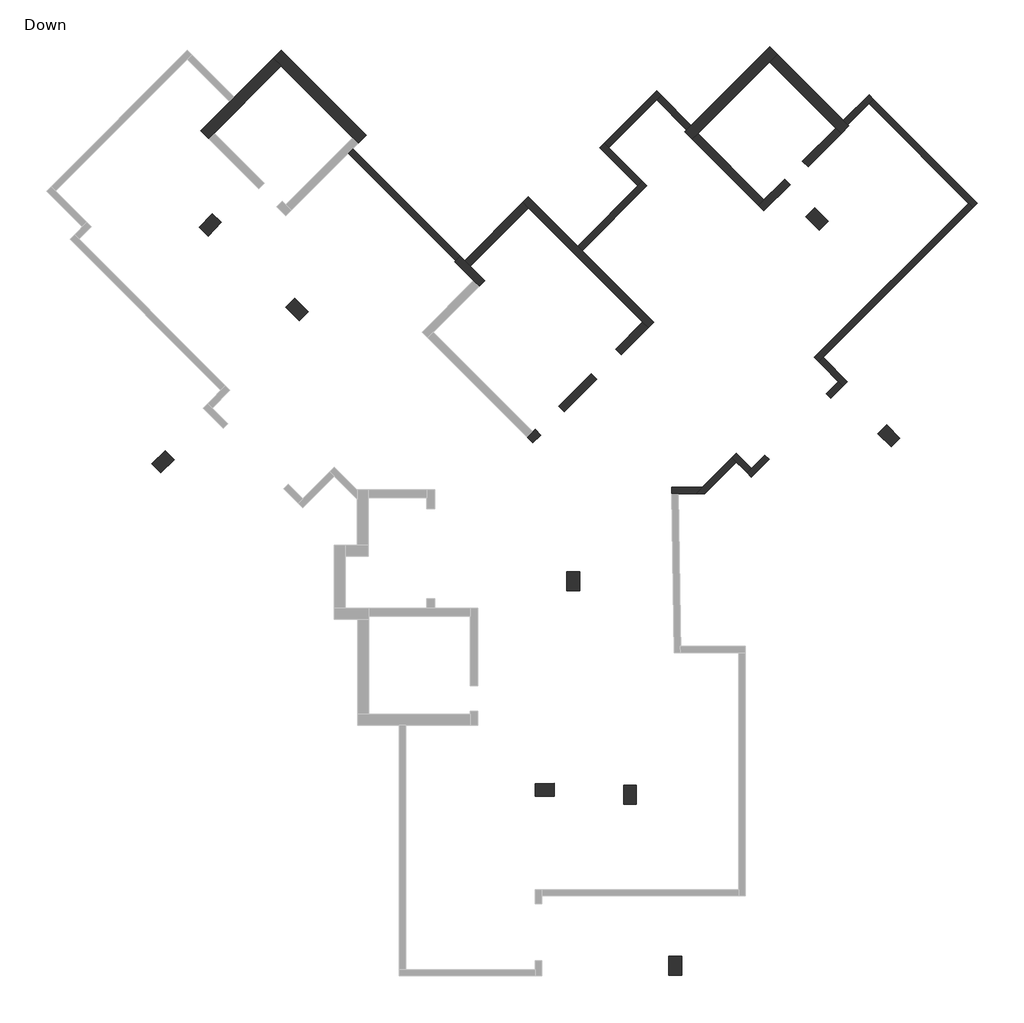
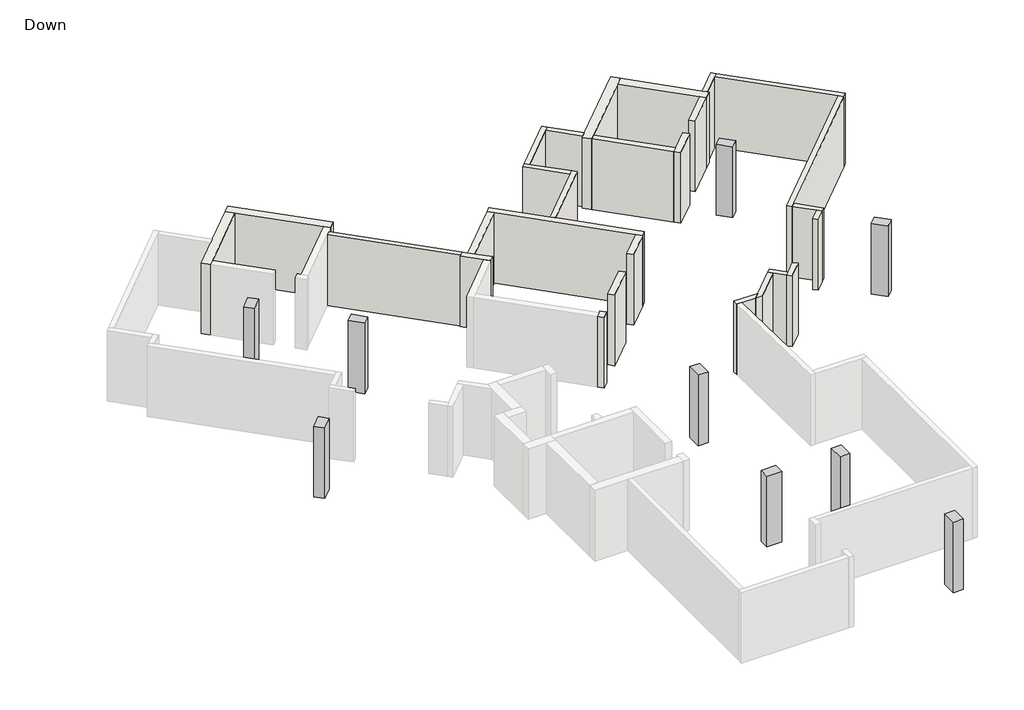
# One storey, part 2 of 2: 27 walls, 9 columns.
"""IFC4 building model written with IfcOpenShell, lengths in millimetres."""

from ifc_helpers import new_model, si_unit, origin, origin_with_axes, place, context, project, spatial, polyline, outline, extrude, faceted_brep, element, save

model = new_model("IFC4")

# Units and contexts
model_context = context("Model", 3, world=origin())
ifc_project = project(units=[si_unit("LENGTHUNIT", "METRE", prefix="MILLI")], contexts=[model_context])

# Site, building, storey
site = spatial("IfcSite", under=ifc_project)
building = spatial("IfcBuilding", under=site)
storey = spatial("IfcBuildingStorey", under=building, Name="Down", Elevation=0.0)

# Columns
placement = place(None, origin())
element("IfcColumn", 1, ObjectType="Concrete Rectengular Column : 40/60", at=placement, inside=storey, context=model_context, shape_type="SweptSolid", body=[
    extrude(outline(polyline([(6112.9804297, -13069.1556852), (6112.9804297, -13669.1556852), (5712.9804297, -13669.1556852), (5712.9804297, -13069.1556852), (6112.9804297, -13069.1556852)])), origin_with_axes(), (0.0, 0.0, 1.0), 3000.0),
])
element("IfcColumn", 2, ObjectType="Concrete Rectengular Column : 40/60", at=placement, inside=storey, context=model_context, shape_type="Brep", body=[
    faceted_brep([(4677.0922421, -7661.9946197, 0.0), (4677.0922421, -8261.9946197, 0.0), (4277.0922421, -8261.9946197, 0.0), (4277.0922421, -7661.9946197, 0.0), (4677.0922421, -7661.9946197, 3000.0), (4677.0922421, -8261.9946197, 3000.0), (4677.0922421, -8261.9946197, 2820.0), (4677.0922421, -7661.9946197, 2820.0), (4277.0922421, -8261.9946197, 3000.0), (4277.0922421, -8261.9946197, 2820.0), (4277.0922421, -7661.9946197, 3000.0), (4277.0922421, -7661.9946197, 2820.0)], [[[0, 1, 2, 3]], [[4, 5, 6, 1, 0, 7]], [[5, 8, 9, 2, 1, 6]], [[8, 10, 11, 3, 2, 9]], [[10, 4, 7, 0, 3, 11]], [[4, 10, 8, 5]]]),
])
element("IfcColumn", 3, ObjectType="Concrete Rectengular Column : 40/60", at=placement, inside=storey, context=model_context, shape_type="Brep", body=[
    faceted_brep([(2484.8469761, -1497.4694814, 0.0), (2484.8469761, -897.4694814, 0.0), (2884.8469761, -897.4694814, 0.0), (2884.8469761, -1497.4694814, 0.0), (2484.8469761, -1497.4694814, 3000.0), (2484.8469761, -897.4694814, 3000.0), (2484.8469761, -897.4694814, 2820.0), (2484.8469761, -1497.4694814, 2820.0), (2884.8469761, -897.4694814, 3000.0), (2884.8469761, -897.4694814, 2820.0), (2884.8469761, -1497.4694814, 3000.0), (2884.8469761, -1497.4694814, 2820.0)], [[[0, 1, 2, 3]], [[4, 5, 6, 1, 0, 7]], [[5, 8, 9, 2, 1, 6]], [[8, 10, 11, 3, 2, 9]], [[10, 4, 7, 0, 3, 11]], [[4, 10, 8, 5]]]),
])
element("IfcColumn", 4, ObjectType="Concrete Rectengular Column : 40/60", at=placement, inside=storey, context=model_context, shape_type="Brep", body=[
    faceted_brep([(-6125.9760682, 7745.4646162, 0.0), (-5702.252807, 7320.6604284, 0.0), (-5985.4555989, 7038.1782543, 0.0), (-6409.17886, 7462.9824421, 0.0), (-6125.9760682, 7745.4646162, 3000.0), (-5702.252807, 7320.6604284, 3000.0), (-5702.252807, 7320.6604284, 2820.0), (-6125.9760682, 7745.4646162, 2820.0), (-5985.4555989, 7038.1782543, 3000.0), (-5985.4555989, 7038.1782543, 2820.0), (-6409.17886, 7462.9824421, 3000.0), (-6409.17886, 7462.9824421, 2820.0)], [[[0, 1, 2, 3]], [[4, 5, 6, 1, 0, 7]], [[5, 8, 9, 2, 1, 6]], [[8, 10, 11, 3, 2, 9]], [[10, 4, 7, 0, 3, 11]], [[4, 10, 8, 5]]]),
])
element("IfcColumn", 5, ObjectType="Concrete Rectengular Column : 40/60", at=placement, inside=storey, context=model_context, shape_type="Brep", body=[
    faceted_brep([(1484.675203, -7607.3508739, 0.0), (2084.6127194, -7598.6919819, 0.0), (2090.385314, -7998.6503262, 0.0), (1490.4477976, -8007.3092182, 0.0), (1484.675203, -7607.3508739, 3000.0), (2084.6127194, -7598.6919819, 3000.0), (2084.6127194, -7598.6919819, 2820.0), (1484.675203, -7607.3508739, 2820.0), (2090.385314, -7998.6503262, 3000.0), (2090.385314, -7998.6503262, 2820.0), (1490.4477976, -8007.3092182, 3000.0), (1490.4477976, -8007.3092182, 2820.0)], [[[0, 1, 2, 3]], [[4, 5, 6, 1, 0, 7]], [[5, 8, 9, 2, 1, 6]], [[8, 10, 11, 3, 2, 9]], [[10, 4, 7, 0, 3, 11]], [[4, 10, 8, 5]]]),
])
element("IfcColumn", 6, ObjectType="Concrete Rectengular Column : 40/60", at=placement, inside=storey, context=model_context, shape_type="Brep", body=[
    faceted_brep([(10319.9156396, 10604.3419273, 0.0), (10744.1797083, 10180.0778586, 0.0), (10461.3369958, 9897.2351461, 0.0), (10037.0729271, 10321.4992148, 0.0), (10319.9156396, 10604.3419273, 3000.0), (10744.1797083, 10180.0778586, 3000.0), (10744.1797083, 10180.0778586, 2820.0), (10319.9156396, 10604.3419273, 2820.0), (10461.3369958, 9897.2351461, 3000.0), (10461.3369958, 9897.2351461, 2820.0), (10037.0729271, 10321.4992148, 3000.0), (10037.0729271, 10321.4992148, 2820.0)], [[[0, 1, 2, 3]], [[4, 5, 6, 1, 0, 7]], [[5, 8, 9, 2, 1, 6]], [[8, 10, 11, 3, 2, 9]], [[10, 4, 7, 0, 3, 11]], [[4, 10, 8, 5]]]),
])
element("IfcColumn", 7, ObjectType="Concrete Rectengular Column : 40/60", at=placement, inside=storey, context=model_context, shape_type="Brep", body=[
    faceted_brep([(-8440.7447422, 10142.7112538, 0.0), (-8856.8048079, 9710.3988417, 0.0), (-9145.0130827, 9987.7722189, 0.0), (-8728.9530169, 10420.084631, 0.0), (-8440.7447422, 10142.7112538, 3000.0), (-8856.8048079, 9710.3988417, 3000.0), (-8856.8048079, 9710.3988417, 2820.0), (-8440.7447422, 10142.7112538, 2820.0), (-9145.0130827, 9987.7722189, 3000.0), (-9145.0130827, 9987.7722189, 2820.0), (-8728.9530169, 10420.084631, 3000.0), (-8728.9530169, 10420.084631, 2820.0)], [[[0, 1, 2, 3]], [[4, 5, 6, 1, 0, 7]], [[5, 8, 9, 2, 1, 6]], [[8, 10, 11, 3, 2, 9]], [[10, 4, 7, 0, 3, 11]], [[4, 10, 8, 5]]]),
])
element("IfcColumn", 8, ObjectType="Concrete Rectengular Column : 40/60", at=placement, inside=storey, context=model_context, shape_type="Brep", body=[
    faceted_brep([(-9937.9307713, 2645.0605261, 0.0), (-10362.7349591, 2221.337265, 0.0), (-10645.2171332, 2504.5400569, 0.0), (-10220.4129454, 2928.263318, 0.0), (-9937.9307713, 2645.0605261, 3000.0), (-10362.7349591, 2221.337265, 3000.0), (-10362.7349591, 2221.337265, 2820.0), (-9937.9307713, 2645.0605261, 2820.0), (-10643.7250884, 2503.0442058, 3000.0), (-10645.2171332, 2504.5400569, 3000.0), (-10220.4129454, 2928.263318, 3000.0), (-10219.2939768, 2927.1414948, 3000.0)], [[[0, 1, 2, 3]], [[4, 5, 6, 1, 0, 7]], [[5, 8, 9, 2, 1, 6]], [[9, 10, 3, 2]], [[10, 11, 4, 7, 0, 3]], [[4, 11, 10, 9, 8, 5]]]),
])
element("IfcColumn", 9, ObjectType="Concrete Rectengular Column : 40/60", at=placement, inside=storey, context=model_context, shape_type="SweptSolid", body=[
    extrude(outline(polyline([(12593.7668598, 3749.362272), (13018.0309285, 3325.0982033), (12735.188216, 3042.2554908), (12310.9241473, 3466.5195596), (12593.7668598, 3749.362272)])), origin_with_axes(), (0.0, 0.0, 1.0), 3000.0),
])

# Walls
element("IfcWall", 10, ObjectType="20", at=placement, inside=storey, context=model_context, shape_type="Brep", body=[
    faceted_brep([(-4429.582499, 12332.1948217, 0.0), (-1033.4026062, 8936.0149288, 0.0), (-1033.4026062, 8936.0149288, 2820.0), (-1033.4026062, 8936.0149288, 3000.0), (-4429.582499, 12332.1948217, 3000.0), (-4429.582499, 12332.1948217, 2820.0), (-4288.1611428, 12473.6161779, 0.0), (-4288.1611428, 12473.6161779, 3000.0), (-891.98125, 9077.4362851, 3000.0), (-891.98125, 9077.4362851, 0.0)], [[[0, 1, 2, 3, 4, 5]], [[6, 7, 8, 9]], [[1, 0, 6, 9]], [[3, 2, 1, 9, 8]], [[4, 3, 8, 7]], [[0, 5, 4, 7, 6]]]),
])
element("IfcWall", 11, ObjectType="20", at=placement, inside=storey, context=model_context, shape_type="Brep", body=[
    faceted_brep([(2962.7877192, 9255.2480262, 0.0), (5013.5473558, 11306.0076628, 0.0), (5013.5473558, 11306.0076628, 2820.0), (5013.5473558, 11306.0076628, 3000.0), (2962.7877192, 9255.2480262, 3000.0), (2962.7877192, 9255.2480262, 2820.0), (2821.3663629, 9396.6693825, 0.0), (2821.3663629, 9396.6693825, 3000.0), (4730.7046433, 11306.0076628, 3000.0), (4872.1259995, 11447.429019, 3000.0), (4872.1259995, 11447.429019, 0.0), (4730.7046433, 11306.0076628, 0.0)], [[[0, 1, 2, 3, 4, 5]], [[6, 7, 8, 9, 10, 11]], [[1, 0, 6, 11, 10]], [[4, 3, 9, 8, 7]], [[0, 5, 4, 7, 6]], [[3, 2, 1, 10, 9]]]),
])
element("IfcWall", 12, ObjectType="20", at=placement, inside=storey, context=model_context, shape_type="Brep", body=[
    faceted_brep([(4872.1259995, 11447.429019, 0.0), (3807.7763909, 12511.7786276, 0.0), (3666.3550347, 12653.1999839, 0.0), (3666.3550347, 12653.1999839, 3000.0), (3807.7763909, 12511.7786276, 3000.0), (4872.1259995, 11447.429019, 3000.0), (4730.7046433, 11306.0076628, 0.0), (4730.7046433, 11306.0076628, 3000.0), (3524.9336785, 12511.7786276, 3000.0), (3524.9336785, 12511.7786276, 0.0)], [[[0, 1, 2, 3, 4, 5]], [[6, 7, 8, 9]], [[2, 1, 0, 6, 9]], [[5, 4, 3, 8, 7]], [[0, 5, 7, 6]], [[3, 2, 9, 8]]]),
])
element("IfcWall", 13, ObjectType="20", at=placement, inside=storey, context=model_context, shape_type="Brep", body=[
    faceted_brep([(3807.7763909, 12511.7786276, 0.0), (5320.554821, 14024.5570577, 0.0), (5461.9761772, 14165.978414, 0.0), (5461.9761772, 14165.978414, 3000.0), (5320.554821, 14024.5570577, 3000.0), (3807.7763909, 12511.7786276, 3000.0), (3807.7763909, 12511.7786276, 2820.0), (3666.3550347, 12653.1999839, 0.0), (3666.3550347, 12653.1999839, 3000.0), (5320.554821, 14307.3997702, 3000.0), (5320.554821, 14307.3997702, 0.0)], [[[0, 1, 2, 3, 4, 5, 6]], [[7, 8, 9, 10]], [[2, 1, 0, 7, 10]], [[5, 4, 3, 9, 8]], [[3, 2, 10, 9]], [[0, 6, 5, 8, 7]]]),
])
element("IfcWall", 14, ObjectType="20", at=placement, inside=storey, context=model_context, shape_type="Brep", body=[
    faceted_brep([(5320.554821, 14024.5570577, 0.0), (6266.9603358, 13078.1515429, 0.0), (6266.9603358, 13078.1515429, 2820.0), (6266.9603358, 13078.1515429, 3000.0), (5320.554821, 14024.5570577, 3000.0), (5320.554821, 14024.5570577, 2820.0), (5461.9761772, 14165.978414, 0.0), (5461.9761772, 14165.978414, 3000.0), (6408.3816921, 13219.5728991, 3000.0), (6408.3816921, 13219.5728991, 0.0)], [[[0, 1, 2, 3, 4, 5]], [[6, 7, 8, 9]], [[1, 0, 6, 9]], [[4, 3, 8, 7]], [[0, 5, 4, 7, 6]], [[3, 2, 1, 9, 8]]]),
])
element("IfcWall", 15, ObjectType="20", at=placement, inside=storey, context=model_context, shape_type="Brep", body=[
    faceted_brep([(11369.6407399, 13231.4427963, 0.0), (12039.7613133, 13901.5633697, 0.0), (12181.1826696, 14042.9847259, 0.0), (12181.1826696, 14042.9847259, 3000.0), (12039.7613133, 13901.5633697, 3000.0), (11369.6407399, 13231.4427963, 3000.0), (11369.6407399, 13231.4427963, 2820.0), (11228.2193837, 13372.8641525, 0.0), (11228.2193837, 13372.8641525, 3000.0), (12039.7613133, 14184.4060822, 3000.0), (12039.7613133, 14184.4060822, 0.0)], [[[0, 1, 2, 3, 4, 5, 6]], [[7, 8, 9, 10]], [[2, 1, 0, 7, 10]], [[5, 4, 3, 9, 8]], [[0, 6, 5, 8, 7]], [[3, 2, 10, 9]]]),
])
element("IfcWall", 16, ObjectType="20", at=placement, inside=storey, context=model_context, shape_type="Brep", body=[
    faceted_brep([(12039.7613133, 13901.5633697, 0.0), (15186.314453, 10755.0102301, 0.0), (15327.7358092, 10613.5888738, 0.0), (15327.7358092, 10613.5888738, 3000.0), (15186.314453, 10755.0102301, 3000.0), (12039.7613133, 13901.5633697, 3000.0), (12039.7613133, 13901.5633697, 2820.0), (12181.1826696, 14042.9847259, 0.0), (12181.1826696, 14042.9847259, 3000.0), (15469.1571655, 10755.0102301, 3000.0), (15469.1571655, 10755.0102301, 0.0)], [[[0, 1, 2, 3, 4, 5, 6]], [[7, 8, 9, 10]], [[2, 1, 0, 7, 10]], [[5, 4, 3, 9, 8]], [[0, 6, 5, 8, 7]], [[3, 2, 10, 9]]]),
])
element("IfcWall", 17, ObjectType="20", at=placement, inside=storey, context=model_context, shape_type="Brep", body=[
    faceted_brep([(15186.314453, 10755.0102301, 0.0), (10305.5209453, 5874.2167224, 0.0), (10305.5209453, 5874.2167224, 2820.0), (10305.5209453, 5874.2167224, 3000.0), (15186.314453, 10755.0102301, 3000.0), (15186.314453, 10755.0102301, 2820.0), (10446.9423016, 5732.7953662, 0.0), (10588.3636578, 5874.2167224, 0.0), (15327.7358092, 10613.5888738, 0.0), (15327.7358092, 10613.5888738, 3000.0), (10588.3636578, 5874.2167224, 3000.0), (10446.9423016, 5732.7953662, 3000.0)], [[[0, 1, 2, 3, 4, 5]], [[6, 7, 8, 9, 10, 11]], [[1, 0, 8, 7, 6]], [[4, 3, 11, 10, 9]], [[0, 5, 4, 9, 8]], [[3, 2, 1, 6, 11]]]),
])
element("IfcWall", 18, ObjectType="20", at=placement, inside=storey, context=model_context, shape_type="Brep", body=[
    faceted_brep([(10446.9423016, 5732.7953662, 0.0), (11069.4524151, 5110.2852526, 0.0), (11210.8737714, 4968.8638964, 0.0), (11210.8737714, 4968.8638964, 3000.0), (11069.4524151, 5110.2852526, 3000.0), (10446.9423016, 5732.7953662, 3000.0), (10588.3636578, 5874.2167224, 0.0), (10588.3636578, 5874.2167224, 3000.0), (11352.2951276, 5110.2852526, 3000.0), (11352.2951276, 5110.2852526, 0.0), (11292.5695034, 5050.5596284, 3000.0)], [[[0, 1, 2, 3, 4, 5]], [[6, 7, 8, 9]], [[2, 1, 0, 6, 9]], [[5, 4, 3, 10, 8, 7]], [[0, 5, 7, 6]], [[3, 2, 9, 8, 10]]]),
])
element("IfcWall", 19, ObjectType="20", at=placement, inside=storey, context=model_context, shape_type="Brep", body=[
    faceted_brep([(11069.4524151, 5110.2852526, 0.0), (10685.5360235, 4726.368861, 0.0), (10685.5360235, 4726.368861, 2820.0), (10685.5360235, 4726.368861, 3000.0), (11069.4524151, 5110.2852526, 3000.0), (11069.4524151, 5110.2852526, 2820.0), (11210.8737714, 4968.8638964, 0.0), (11210.8737714, 4968.8638964, 3000.0), (10826.9573797, 4584.9475048, 3000.0), (10826.9573797, 4584.9475048, 2820.0), (10826.9573797, 4584.9475048, 0.0)], [[[0, 1, 2, 3, 4, 5]], [[6, 7, 8, 9, 10]], [[1, 0, 6, 10]], [[3, 2, 1, 10, 9, 8]], [[4, 3, 8, 7]], [[0, 5, 4, 7, 6]]]),
])
element("IfcWall", 20, ObjectType="20", at=placement, inside=storey, context=model_context, shape_type="Brep", body=[
    faceted_brep([(8747.3931582, 2788.2259957, 0.0), (8323.1290895, 2363.961927, 0.0), (8181.7077332, 2222.5405707, 0.0), (8181.7077332, 2222.5405707, 3000.0), (8323.1290895, 2363.961927, 3000.0), (8747.3931582, 2788.2259957, 3000.0), (8747.3931582, 2788.2259957, 2820.0), (8888.8145144, 2646.8046394, 0.0), (8888.8145144, 2646.8046394, 2820.0), (8888.8145144, 2646.8046394, 3000.0), (8393.4317005, 2151.4218256, 3000.0), (8323.1290895, 2081.1192145, 3000.0), (8323.1290895, 2081.1192145, 0.0)], [[[0, 1, 2, 3, 4, 5, 6]], [[7, 8, 9, 10, 11, 12]], [[2, 1, 0, 7, 12]], [[5, 4, 3, 11, 10, 9]], [[0, 6, 5, 9, 8, 7]], [[3, 2, 12, 11]]]),
])
element("IfcWall", 21, ObjectType="20", at=placement, inside=storey, context=model_context, shape_type="Brep", body=[
    faceted_brep([(8323.1290895, 2363.961927, 0.0), (7842.9320868, 2844.1589296, 0.0), (7842.9320868, 2844.1589296, 2820.0), (7842.9320868, 2844.1589296, 3000.0), (8323.1290895, 2363.961927, 3000.0), (8323.1290895, 2363.961927, 2820.0), (8181.7077332, 2222.5405707, 0.0), (8181.7077332, 2222.5405707, 3000.0), (7842.9320868, 2561.3162171, 3000.0), (7701.5107306, 2702.7375734, 3000.0), (7701.5107306, 2702.7375734, 0.0), (7842.9320868, 2561.3162171, 0.0)], [[[0, 1, 2, 3, 4, 5]], [[6, 7, 8, 9, 10, 11]], [[1, 0, 6, 11, 10]], [[4, 3, 9, 8, 7]], [[0, 5, 4, 7, 6]], [[3, 2, 1, 10, 9]]]),
])
element("IfcWall", 22, ObjectType="20", at=placement, inside=storey, context=model_context, shape_type="Brep", body=[
    faceted_brep([(7701.5107306, 2702.7375734, 0.0), (6767.6697714, 1768.8966142, 0.0), (6567.6697714, 1568.8966142, 0.0), (6567.6697714, 1568.8966142, 3000.0), (6767.6697714, 1768.8966142, 3000.0), (7701.5107306, 2702.7375734, 3000.0), (7842.9320868, 2561.3162171, 0.0), (7842.9320868, 2561.3162171, 3000.0), (6850.5124839, 1568.8966142, 3000.0), (6850.5124839, 1568.8966142, 0.0)], [[[0, 1, 2, 3, 4, 5]], [[6, 7, 8, 9]], [[2, 1, 0, 6, 9]], [[5, 4, 3, 8, 7]], [[0, 5, 7, 6]], [[3, 2, 9, 8]]]),
])
element("IfcWall", 23, ObjectType="20", at=placement, inside=storey, context=model_context, shape_type="Brep", body=[
    faceted_brep([(6767.6697714, 1768.8966142, 0.0), (5805.6765523, 1768.8966142, 0.0), (5805.6765523, 1768.8966142, 2820.0), (5805.6765523, 1768.8966142, 3000.0), (6767.6697714, 1768.8966142, 3000.0), (6767.6697714, 1768.8966142, 2820.0), (6567.6697714, 1568.8966142, 0.0), (6567.6697714, 1568.8966142, 3000.0), (6008.5087812, 1568.8966142, 3000.0), (5808.4890075, 1568.8966142, 3000.0), (5808.4890075, 1568.8966142, 0.0), (6008.5087812, 1568.8966142, 0.0)], [[[0, 1, 2, 3, 4, 5]], [[6, 7, 8, 9, 10, 11]], [[1, 0, 6, 11, 10]], [[4, 3, 9, 8, 7]], [[0, 5, 4, 7, 6]], [[3, 2, 1, 10, 9]]]),
])
element("IfcWall", 24, ObjectType="25", at=placement, inside=storey, context=model_context, shape_type="Brep", body=[
    faceted_brep([(10980.691113, 13125.4176764, 0.0), (9934.0396226, 12078.766186, 0.0), (9934.0396226, 12078.766186, 2820.0), (9934.0396226, 12078.766186, 3000.0), (10980.691113, 13125.4176764, 3000.0), (10980.691113, 13125.4176764, 2820.0), (11157.4678083, 12948.6409811, 0.0), (11157.4678083, 12948.6409811, 3000.0), (10110.8163179, 11901.9894907, 3000.0), (10110.8163179, 11901.9894907, 2820.0), (10110.8163179, 11901.9894907, 0.0)], [[[0, 1, 2, 3, 4, 5]], [[6, 7, 8, 9, 10]], [[1, 0, 6, 10]], [[3, 2, 1, 10, 9, 8]], [[4, 3, 8, 7]], [[0, 5, 4, 7, 6]]]),
])
element("IfcWall", 25, ObjectType="25", at=placement, inside=storey, context=model_context, shape_type="Brep", body=[
    faceted_brep([(8717.8496812, 10509.0228541, 0.0), (9546.3438201, 11337.5169929, 0.0), (9546.3438201, 11337.5169929, 2820.0), (9546.3438201, 11337.5169929, 3000.0), (8717.8496812, 10509.0228541, 3000.0), (8717.8496812, 10509.0228541, 2820.0), (8541.0729859, 10685.7995493, 0.0), (8541.0729859, 10685.7995493, 3000.0), (8717.8496812, 10862.5762446, 3000.0), (9369.5671248, 11514.2936882, 3000.0), (9369.5671248, 11514.2936882, 2820.0), (9369.5671248, 11514.2936882, 0.0), (8717.8496812, 10862.5762446, 0.0)], [[[0, 1, 2, 3, 4, 5]], [[6, 7, 8, 9, 10, 11, 12]], [[1, 0, 6, 12, 11]], [[3, 2, 1, 11, 10, 9]], [[4, 3, 9, 8, 7]], [[0, 5, 4, 7, 6]]]),
])
element("IfcWall", 26, ObjectType="25", at=placement, inside=storey, context=model_context, shape_type="Brep", body=[
    faceted_brep([(8717.8496812, 10862.5762446, 0.0), (6632.1047328, 12948.3211931, 0.0), (6632.1047328, 12948.3211931, 2820.0), (6632.1047328, 12948.3211931, 3000.0), (8717.8496812, 10862.5762446, 3000.0), (8717.8496812, 10862.5762446, 2820.0), (8541.0729859, 10685.7995493, 0.0), (8541.0729859, 10685.7995493, 3000.0), (6455.3280375, 12771.5444978, 3000.0), (6455.3280375, 12771.5444978, 0.0)], [[[0, 1, 2, 3, 4, 5]], [[6, 7, 8, 9]], [[1, 0, 6, 9]], [[4, 3, 8, 7]], [[3, 2, 1, 9, 8]], [[0, 5, 4, 7, 6]]]),
])
element("IfcWall", 27, ObjectType="25", at=placement, inside=storey, context=model_context, shape_type="Brep", body=[
    faceted_brep([(5227.1373278, 6990.8984176, 0.0), (2962.7877192, 9255.2480262, 0.0), (2821.3663629, 9396.6693825, 0.0), (1265.7304614, 10952.305284, 0.0), (1265.7304614, 10952.305284, 3000.0), (2821.3663629, 9396.6693825, 3000.0), (2962.7877192, 9255.2480262, 3000.0), (5227.1373278, 6990.8984176, 3000.0), (5227.1373278, 6990.8984176, 2820.0), (5050.3606325, 6814.1217223, 0.0), (5050.3606325, 6814.1217223, 3000.0), (4873.5839372, 6990.8984176, 3000.0), (1265.7304614, 10598.7518934, 3000.0), (1088.9537661, 10775.5285887, 3000.0), (1088.9537661, 10775.5285887, 0.0), (1265.7304614, 10598.7518934, 0.0), (4873.5839372, 6990.8984176, 0.0)], [[[0, 1, 2, 3, 4, 5, 6, 7, 8]], [[9, 10, 11, 12, 13, 14, 15, 16]], [[3, 2, 1, 0, 9, 16, 15, 14]], [[7, 6, 5, 4, 13, 12, 11, 10]], [[4, 3, 14, 13]], [[0, 8, 7, 10, 9]]]),
])
element("IfcWall", 28, ObjectType="25", at=placement, inside=storey, context=model_context, shape_type="SweptSolid", body=[
    extrude(outline(polyline([(-750.5003772, 8936.0744454), (1088.9537661, 10775.5285887), (1265.7304614, 10598.7518934), (-573.7236819, 8759.2977501), (-750.5003772, 8936.0744454)])), origin_with_axes(), (0.0, 0.0, 1.0), 3000.0),
])
element("IfcWall", 29, ObjectType="25", at=placement, inside=storey, context=model_context, shape_type="Brep", body=[
    faceted_brep([(-115.3333666, 8300.9074348, 0.0), (-573.7236819, 8759.2977501, 0.0), (-750.5003772, 8936.0744454, 0.0), (-891.9217334, 9077.4958016, 0.0), (-891.9217334, 9077.4958016, 3000.0), (-750.5003772, 8936.0744454, 3000.0), (-573.7236819, 8759.2977501, 3000.0), (-115.3333666, 8300.9074348, 3000.0), (-292.1100618, 8124.1307395, 0.0), (-292.1100618, 8124.1307395, 3000.0), (-468.8867571, 8300.9074348, 3000.0), (-1068.6984287, 8900.7191063, 3000.0), (-1068.6984287, 8900.7191063, 2820.0), (-1068.6984287, 8900.7191063, 0.0), (-468.8867571, 8300.9074348, 0.0), (-1033.4026062, 8936.0149288, 0.0), (-1033.4026062, 8936.0149288, 3000.0)], [[[0, 1, 2, 3, 4, 5, 6, 7]], [[8, 9, 10, 11, 12, 13, 14]], [[3, 2, 1, 0, 8, 14, 13, 15]], [[4, 3, 15, 13, 12, 11, 16]], [[7, 6, 5, 4, 16, 11, 10, 9]], [[0, 7, 9, 8]]]),
])
element("IfcWall", 30, ObjectType="25", at=placement, inside=storey, context=model_context, shape_type="Brep", body=[
    faceted_brep([(1407.8225017, 3171.5835916, 0.0), (1655.2707813, 3419.0318712, 0.0), (1655.2707813, 3419.0318712, 2820.0), (1655.2707813, 3419.0318712, 3000.0), (1407.8225017, 3171.5835916, 3000.0), (1407.8225017, 3171.5835916, 2820.0), (1231.0458064, 3348.3602869, 0.0), (1231.0458064, 3348.3602869, 3000.0), (1407.8225017, 3525.1369821, 3000.0), (1478.494086, 3595.8085665, 3000.0), (1478.494086, 3595.8085665, 2820.0), (1478.494086, 3595.8085665, 0.0), (1407.8225017, 3525.1369821, 0.0)], [[[0, 1, 2, 3, 4, 5]], [[6, 7, 8, 9, 10, 11, 12]], [[1, 0, 6, 12, 11]], [[3, 2, 1, 11, 10, 9]], [[4, 3, 9, 8, 7]], [[0, 5, 4, 7, 6]]]),
])
element("IfcWall", 31, ObjectType="25", at=placement, inside=storey, context=model_context, shape_type="Brep", body=[
    faceted_brep([(2397.561133, 4161.3222229, 0.0), (3424.432188, 5188.1932779, 0.0), (3424.432188, 5188.1932779, 2820.0), (3424.432188, 5188.1932779, 3000.0), (2397.561133, 4161.3222229, 3000.0), (2397.561133, 4161.3222229, 2820.0), (2220.7844377, 4338.0989181, 0.0), (2220.7844377, 4338.0989181, 2820.0), (2220.7844377, 4338.0989181, 3000.0), (3247.6554927, 5364.9699732, 3000.0), (3247.6554927, 5364.9699732, 2820.0), (3247.6554927, 5364.9699732, 0.0)], [[[0, 1, 2, 3, 4, 5]], [[6, 7, 8, 9, 10, 11]], [[1, 0, 6, 11]], [[3, 2, 1, 11, 10, 9]], [[4, 3, 9, 8]], [[0, 5, 4, 8, 7, 6]]]),
])
element("IfcWall", 32, ObjectType="25", at=placement, inside=storey, context=model_context, shape_type="Brep", body=[
    faceted_brep([(4199.1842169, 5962.9453067, 0.0), (5050.3606325, 6814.1217223, 0.0), (5050.3606325, 6814.1217223, 3000.0), (4199.1842169, 5962.9453067, 3000.0), (4199.1842169, 5962.9453067, 2820.0), (4022.4075216, 6139.722002, 0.0), (4022.4075216, 6139.722002, 2820.0), (4022.4075216, 6139.722002, 3000.0), (4873.5839372, 6990.8984176, 3000.0), (4873.5839372, 6990.8984176, 0.0)], [[[0, 1, 2, 3, 4]], [[5, 6, 7, 8, 9]], [[1, 0, 5, 9]], [[3, 2, 8, 7]], [[0, 4, 3, 7, 6, 5]], [[2, 1, 9, 8]]]),
])
element("IfcWall", 33, ObjectType="35", at=placement, inside=storey, context=model_context, shape_type="Brep", body=[
    faceted_brep([(-6797.446529, 15338.5417926, 0.0), (-6549.9591555, 15091.0544192, 0.0), (-4287.1177238, 12828.2129875, 0.0), (-4110.3410285, 12651.4362922, 0.0), (-4110.3410285, 12651.4362922, 3000.0), (-4287.1177238, 12828.2129875, 3000.0), (-6549.9591555, 15091.0544192, 3000.0), (-6797.446529, 15338.5417926, 3000.0), (-6549.9591555, 15586.029166, 0.0), (-6549.9591555, 15586.029166, 3000.0), (-3862.8536551, 12898.9236656, 3000.0), (-3862.8536551, 12898.9236656, 0.0)], [[[0, 1, 2, 3, 4, 5, 6, 7]], [[8, 9, 10, 11]], [[3, 2, 1, 0, 8, 11]], [[7, 6, 5, 4, 10, 9]], [[0, 7, 9, 8]], [[4, 3, 11, 10]]]),
])
element("IfcWall", 34, ObjectType="35", at=placement, inside=storey, context=model_context, shape_type="Brep", body=[
    faceted_brep([(-6797.446529, 15338.5417926, 0.0), (-8031.9823439, 14104.0059776, 0.0), (-8173.4037002, 13962.5846214, 0.0), (-9095.6760176, 13040.312304, 0.0), (-9095.6760176, 13040.312304, 2820.0), (-9095.6760176, 13040.312304, 3000.0), (-8173.4037002, 13962.5846214, 3000.0), (-8031.9823439, 14104.0059776, 3000.0), (-6797.446529, 15338.5417926, 3000.0), (-6549.9591555, 15091.0544192, 0.0), (-6549.9591555, 15091.0544192, 2820.0), (-6549.9591555, 15091.0544192, 3000.0), (-8671.4119489, 12969.6016259, 3000.0), (-8848.1886442, 12792.8249306, 3000.0), (-8848.1886442, 12792.8249306, 0.0), (-8671.4119489, 12969.6016259, 0.0)], [[[0, 1, 2, 3, 4, 5, 6, 7, 8]], [[9, 10, 11, 12, 13, 14, 15]], [[3, 2, 1, 0, 9, 15, 14]], [[8, 7, 6, 5, 13, 12, 11]], [[0, 8, 11, 10, 9]], [[5, 4, 3, 14, 13]]]),
])
element("IfcWall", 35, ObjectType="35", at=placement, inside=storey, context=model_context, shape_type="Brep", body=[
    faceted_brep([(6455.3280375, 12771.5444978, 0.0), (6632.1047328, 12948.3211931, 0.0), (8894.9461646, 15211.1626248, 0.0), (9142.433538, 15458.6499982, 0.0), (9142.433538, 15458.6499982, 3000.0), (8894.9461646, 15211.1626248, 3000.0), (6632.1047328, 12948.3211931, 3000.0), (6455.3280375, 12771.5444978, 3000.0), (6207.8406641, 13019.0318712, 0.0), (6207.8406641, 13019.0318712, 2820.0), (6207.8406641, 13019.0318712, 3000.0), (6266.9603358, 13078.1515429, 3000.0), (6408.3816921, 13219.5728991, 3000.0), (8894.9461646, 15706.1373716, 3000.0), (8894.9461646, 15706.1373716, 0.0), (6408.3816921, 13219.5728991, 0.0), (6266.9603358, 13078.1515429, 0.0)], [[[0, 1, 2, 3, 4, 5, 6, 7]], [[8, 9, 10, 11, 12, 13, 14, 15, 16]], [[3, 2, 1, 0, 8, 16, 15, 14]], [[7, 6, 5, 4, 13, 12, 11, 10]], [[4, 3, 14, 13]], [[0, 7, 10, 9, 8]]]),
])
element("IfcWall", 36, ObjectType="35", at=placement, inside=storey, context=model_context, shape_type="Brep", body=[
    faceted_brep([(8894.9461646, 15211.1626248, 0.0), (10980.691113, 13125.4176764, 0.0), (11157.4678083, 12948.6409811, 0.0), (11157.4678083, 12948.6409811, 3000.0), (10980.691113, 13125.4176764, 3000.0), (8894.9461646, 15211.1626248, 3000.0), (8894.9461646, 15211.1626248, 2820.0), (9142.433538, 15458.6499982, 0.0), (9142.433538, 15458.6499982, 3000.0), (11228.2193837, 13372.8641525, 3000.0), (11369.6407399, 13231.4427963, 3000.0), (11404.9551817, 13196.1283545, 3000.0), (11404.9551817, 13196.1283545, 2820.0), (11404.9551817, 13196.1283545, 0.0), (11369.6407399, 13231.4427963, 0.0), (11228.2193837, 13372.8641525, 0.0)], [[[0, 1, 2, 3, 4, 5, 6]], [[7, 8, 9, 10, 11, 12, 13, 14, 15]], [[2, 1, 0, 7, 15, 14, 13]], [[5, 4, 3, 11, 10, 9, 8]], [[0, 6, 5, 8, 7]], [[3, 2, 13, 12, 11]]]),
])

save(model, "model.ifc")

# Revit data of these elements
# Type "Concrete Rectengular Column : 40/60"
#   b = 40 cm
#   h = 60 cm
#   Structural Material [instance default] = Concrete
# Type "20"
#   Layers, outside or top first: 20 cm "Concrete" (function 1)
# Type "25"
#   Layers, outside or top first: 25 cm "Concrete" (function 1)
# Type "35"
#   Layers, outside or top first: 35 cm "Concrete" (function 1)
# Element 1 (IfcColumn, "Concrete Rectengular Column : 40/60")
#   Comments = ""
#   Mark = "C1"
#   SOFiSTiK_AMG_Comments = ""
#   SOFiSTiK_AMG_Scheduled = yes
#   SOFiSTiK_AMG_Adjusted = yes
#   Structural Material = Concrete
#   Phase Created = New Construction
#   Materials on its faces: "Concrete"
# Element 2 (IfcColumn, "Concrete Rectengular Column : 40/60")
#   Comments = ""
#   Mark = "C2"
#   SOFiSTiK_AMG_Comments = ""
#   SOFiSTiK_AMG_Scheduled = yes
#   SOFiSTiK_AMG_Adjusted = yes
#   Structural Material = Concrete
#   Phase Created = New Construction
#   Materials on its faces: "Concrete"
# Element 3 (IfcColumn, "Concrete Rectengular Column : 40/60")
#   Comments = ""
#   Mark = "C3"
#   SOFiSTiK_AMG_Comments = ""
#   SOFiSTiK_AMG_Scheduled = yes
#   SOFiSTiK_AMG_Adjusted = yes
#   Structural Material = Concrete
#   Phase Created = New Construction
#   Materials on its faces: "Concrete"
# Element 4 (IfcColumn, "Concrete Rectengular Column : 40/60")
#   Comments = ""
#   Mark = "C4"
#   SOFiSTiK_AMG_Comments = ""
#   SOFiSTiK_AMG_Scheduled = yes
#   SOFiSTiK_AMG_Adjusted = yes
#   Structural Material = Concrete
#   Phase Created = New Construction
#   Materials on its faces: "Concrete"
# Element 5 (IfcColumn, "Concrete Rectengular Column : 40/60")
#   Comments = ""
#   Mark = "C5"
#   SOFiSTiK_AMG_Comments = ""
#   SOFiSTiK_AMG_Scheduled = yes
#   SOFiSTiK_AMG_Adjusted = yes
#   Structural Material = Concrete
#   Phase Created = New Construction
#   Materials on its faces: "Concrete"
# Element 6 (IfcColumn, "Concrete Rectengular Column : 40/60")
#   Comments = ""
#   Mark = "C6"
#   SOFiSTiK_AMG_Comments = ""
#   SOFiSTiK_AMG_Scheduled = yes
#   SOFiSTiK_AMG_Adjusted = yes
#   Structural Material = Concrete
#   Phase Created = New Construction
#   Materials on its faces: "Concrete"
# Element 7 (IfcColumn, "Concrete Rectengular Column : 40/60")
#   Comments = ""
#   Mark = "C7"
#   SOFiSTiK_AMG_Comments = ""
#   SOFiSTiK_AMG_Scheduled = yes
#   SOFiSTiK_AMG_Adjusted = yes
#   Structural Material = Concrete
#   Phase Created = New Construction
#   Materials on its faces: "Concrete"
# Element 8 (IfcColumn, "Concrete Rectengular Column : 40/60")
#   Comments = ""
#   Mark = "C8"
#   SOFiSTiK_AMG_Comments = ""
#   SOFiSTiK_AMG_Scheduled = yes
#   SOFiSTiK_AMG_Adjusted = yes
#   Structural Material = Concrete
#   Phase Created = New Construction
#   Materials on its faces: "Concrete"
# Element 9 (IfcColumn, "Concrete Rectengular Column : 40/60")
#   Comments = ""
#   Mark = "C9"
#   SOFiSTiK_AMG_Comments = ""
#   SOFiSTiK_AMG_Scheduled = yes
#   SOFiSTiK_AMG_Adjusted = yes
#   Structural Material = Concrete
#   Phase Created = New Construction
#   Materials on its faces: "Concrete"
# Element 10 (IfcWall, "20")
#   Comments = ""
#   Mark = "W41"
#   SOFiSTiK_EdgeZones = "W41"
#   SOFiSTiK_AMG_Comments = ""
#   Top Offset = 0 cm
#   Base Offset = 0 cm
#   wall height = 300 cm
#   SOFiSTiK_AMG_Scheduled = yes
#   SOFiSTiK_AMG_Adjusted = yes
#   Phase Created = New Construction
#   Base Constraint = Down
#   Top Constraint = Typical Floor
#   Materials on its faces: "Concrete"
# Element 11 (IfcWall, "20")
#   Comments = ""
#   Mark = "W42"
#   SOFiSTiK_EdgeZones = "W42"
#   SOFiSTiK_AMG_Comments = ""
#   Top Offset = 0 cm
#   Base Offset = 0 cm
#   wall height = 300 cm
#   SOFiSTiK_AMG_Scheduled = yes
#   SOFiSTiK_AMG_Adjusted = yes
#   Phase Created = New Construction
#   Base Constraint = Down
#   Top Constraint = Typical Floor
#   Materials on its faces: "Concrete"
# Element 12 (IfcWall, "20")
#   Comments = ""
#   Mark = "W43"
#   SOFiSTiK_EdgeZones = "W43"
#   SOFiSTiK_AMG_Comments = ""
#   Top Offset = 0 cm
#   Base Offset = 0 cm
#   wall height = 300 cm
#   SOFiSTiK_AMG_Scheduled = yes
#   SOFiSTiK_AMG_Adjusted = yes
#   Phase Created = New Construction
#   Base Constraint = Down
#   Top Constraint = Typical Floor
#   Materials on its faces: "Concrete"
# Element 13 (IfcWall, "20")
#   Comments = ""
#   Mark = "W44"
#   SOFiSTiK_EdgeZones = "W44"
#   SOFiSTiK_AMG_Comments = ""
#   Top Offset = 0 cm
#   Base Offset = 0 cm
#   wall height = 300 cm
#   SOFiSTiK_AMG_Scheduled = yes
#   SOFiSTiK_AMG_Adjusted = yes
#   Phase Created = New Construction
#   Base Constraint = Down
#   Top Constraint = Typical Floor
#   Materials on its faces: "Concrete"
# Element 14 (IfcWall, "20")
#   Comments = ""
#   Mark = "W45"
#   SOFiSTiK_EdgeZones = "W45"
#   SOFiSTiK_AMG_Comments = ""
#   Top Offset = 0 cm
#   Base Offset = 0 cm
#   wall height = 300 cm
#   SOFiSTiK_AMG_Scheduled = yes
#   SOFiSTiK_AMG_Adjusted = yes
#   Phase Created = New Construction
#   Base Constraint = Down
#   Top Constraint = Typical Floor
#   Materials on its faces: "Concrete"
# Element 15 (IfcWall, "20")
#   Comments = ""
#   Mark = "W46"
#   SOFiSTiK_EdgeZones = "W46"
#   SOFiSTiK_AMG_Comments = ""
#   Top Offset = 0 cm
#   Base Offset = 0 cm
#   wall height = 300 cm
#   SOFiSTiK_AMG_Scheduled = yes
#   SOFiSTiK_AMG_Adjusted = yes
#   Phase Created = New Construction
#   Base Constraint = Down
#   Top Constraint = Typical Floor
#   Materials on its faces: "Concrete"
# Element 16 (IfcWall, "20")
#   Comments = ""
#   Mark = "W47"
#   SOFiSTiK_EdgeZones = "W47"
#   SOFiSTiK_AMG_Comments = ""
#   Top Offset = 0 cm
#   Base Offset = 0 cm
#   wall height = 300 cm
#   SOFiSTiK_AMG_Scheduled = yes
#   SOFiSTiK_AMG_Adjusted = yes
#   Phase Created = New Construction
#   Base Constraint = Down
#   Top Constraint = Typical Floor
#   Materials on its faces: "Concrete"
# Element 17 (IfcWall, "20")
#   Comments = ""
#   Mark = "W48"
#   SOFiSTiK_EdgeZones = "W48"
#   SOFiSTiK_AMG_Comments = ""
#   Top Offset = 0 cm
#   Base Offset = 0 cm
#   wall height = 300 cm
#   SOFiSTiK_AMG_Scheduled = yes
#   SOFiSTiK_AMG_Adjusted = yes
#   Phase Created = New Construction
#   Base Constraint = Down
#   Top Constraint = Typical Floor
#   Materials on its faces: "Concrete"
# Element 18 (IfcWall, "20")
#   Comments = ""
#   Mark = "W49"
#   SOFiSTiK_EdgeZones = "W49"
#   SOFiSTiK_AMG_Comments = ""
#   Top Offset = 0 cm
#   Base Offset = 0 cm
#   wall height = 300 cm
#   SOFiSTiK_AMG_Scheduled = yes
#   SOFiSTiK_AMG_Adjusted = yes
#   Phase Created = New Construction
#   Base Constraint = Down
#   Top Constraint = Typical Floor
#   Materials on its faces: "Concrete"
# Element 19 (IfcWall, "20")
#   Comments = ""
#   Mark = "W50"
#   SOFiSTiK_EdgeZones = "W50"
#   SOFiSTiK_AMG_Comments = ""
#   Top Offset = 0 cm
#   Base Offset = 0 cm
#   wall height = 300 cm
#   SOFiSTiK_AMG_Scheduled = yes
#   SOFiSTiK_AMG_Adjusted = yes
#   Phase Created = New Construction
#   Base Constraint = Down
#   Top Constraint = Typical Floor
#   Materials on its faces: "Concrete"
# Element 20 (IfcWall, "20")
#   Comments = ""
#   Mark = "W51"
#   SOFiSTiK_EdgeZones = "W51"
#   SOFiSTiK_AMG_Comments = ""
#   Top Offset = 0 cm
#   Base Offset = 0 cm
#   wall height = 300 cm
#   SOFiSTiK_AMG_Scheduled = yes
#   SOFiSTiK_AMG_Adjusted = yes
#   Phase Created = New Construction
#   Base Constraint = Down
#   Top Constraint = Typical Floor
#   Materials on its faces: "Concrete"
# Element 21 (IfcWall, "20")
#   Comments = ""
#   Mark = "W52"
#   SOFiSTiK_EdgeZones = "W52"
#   SOFiSTiK_AMG_Comments = ""
#   Top Offset = 0 cm
#   Base Offset = 0 cm
#   wall height = 300 cm
#   SOFiSTiK_AMG_Scheduled = yes
#   SOFiSTiK_AMG_Adjusted = yes
#   Phase Created = New Construction
#   Base Constraint = Down
#   Top Constraint = Typical Floor
#   Materials on its faces: "Concrete"
# Element 22 (IfcWall, "20")
#   Comments = ""
#   Mark = "W53"
#   SOFiSTiK_EdgeZones = "W53"
#   SOFiSTiK_AMG_Comments = ""
#   Top Offset = 0 cm
#   Base Offset = 0 cm
#   wall height = 300 cm
#   SOFiSTiK_AMG_Scheduled = yes
#   SOFiSTiK_AMG_Adjusted = yes
#   Phase Created = New Construction
#   Base Constraint = Down
#   Top Constraint = Typical Floor
#   Materials on its faces: "Concrete"
# Element 23 (IfcWall, "20")
#   Comments = ""
#   Mark = "W54"
#   SOFiSTiK_EdgeZones = "W54"
#   SOFiSTiK_AMG_Comments = ""
#   Top Offset = 0 cm
#   Base Offset = 0 cm
#   wall height = 300 cm
#   SOFiSTiK_AMG_Scheduled = yes
#   SOFiSTiK_AMG_Adjusted = yes
#   Phase Created = New Construction
#   Base Constraint = Down
#   Top Constraint = Typical Floor
#   Materials on its faces: "Concrete"
# Element 24 (IfcWall, "25")
#   Comments = ""
#   Mark = "W14"
#   SOFiSTiK_EdgeZones = "W14"
#   SOFiSTiK_AMG_Comments = ""
#   Top Offset = 0 cm
#   Base Offset = 0 cm
#   wall height = 300 cm
#   SOFiSTiK_AMG_Scheduled = yes
#   SOFiSTiK_AMG_Adjusted = yes
#   Phase Created = New Construction
#   Base Constraint = Down
#   Top Constraint = Typical Floor
#   Materials on its faces: "Concrete"
# Element 25 (IfcWall, "25")
#   Comments = ""
#   Mark = "W15"
#   SOFiSTiK_EdgeZones = "W15"
#   SOFiSTiK_AMG_Comments = ""
#   Top Offset = 0 cm
#   Base Offset = 0 cm
#   wall height = 300 cm
#   SOFiSTiK_AMG_Scheduled = yes
#   SOFiSTiK_AMG_Adjusted = yes
#   Phase Created = New Construction
#   Base Constraint = Down
#   Top Constraint = Typical Floor
#   Materials on its faces: "Concrete"
# Element 26 (IfcWall, "25")
#   Comments = ""
#   Mark = "W16"
#   SOFiSTiK_EdgeZones = "W16"
#   SOFiSTiK_AMG_Comments = ""
#   Top Offset = 0 cm
#   Base Offset = 0 cm
#   wall height = 300 cm
#   SOFiSTiK_AMG_Scheduled = yes
#   SOFiSTiK_AMG_Adjusted = yes
#   Phase Created = New Construction
#   Base Constraint = Down
#   Top Constraint = Typical Floor
#   Materials on its faces: "Concrete"
# Element 27 (IfcWall, "25")
#   Comments = ""
#   Mark = "W17"
#   SOFiSTiK_EdgeZones = "W17"
#   SOFiSTiK_AMG_Comments = ""
#   Top Offset = 0 cm
#   Base Offset = 0 cm
#   wall height = 300 cm
#   SOFiSTiK_AMG_Scheduled = yes
#   SOFiSTiK_AMG_Adjusted = yes
#   Phase Created = New Construction
#   Base Constraint = Down
#   Top Constraint = Typical Floor
#   Materials on its faces: "Concrete"
# Element 28 (IfcWall, "25")
#   Comments = ""
#   Mark = "W18"
#   SOFiSTiK_EdgeZones = "W18"
#   SOFiSTiK_AMG_Comments = ""
#   Top Offset = 0 cm
#   Base Offset = 0 cm
#   wall height = 300 cm
#   SOFiSTiK_AMG_Scheduled = yes
#   SOFiSTiK_AMG_Adjusted = yes
#   Phase Created = New Construction
#   Base Constraint = Down
#   Top Constraint = Typical Floor
#   Materials on its faces: "Concrete"
# Element 29 (IfcWall, "25")
#   Comments = ""
#   Mark = "W19"
#   SOFiSTiK_EdgeZones = "W19"
#   SOFiSTiK_AMG_Comments = ""
#   Top Offset = 0 cm
#   Base Offset = 0 cm
#   wall height = 300 cm
#   SOFiSTiK_AMG_Scheduled = yes
#   SOFiSTiK_AMG_Adjusted = yes
#   Phase Created = New Construction
#   Base Constraint = Down
#   Top Constraint = Typical Floor
#   Materials on its faces: "Concrete"
# Element 30 (IfcWall, "25")
#   Comments = ""
#   Mark = "W22"
#   SOFiSTiK_EdgeZones = "W22"
#   SOFiSTiK_AMG_Comments = ""
#   Top Offset = 0 cm
#   Base Offset = 0 cm
#   wall height = 300 cm
#   SOFiSTiK_AMG_Scheduled = yes
#   SOFiSTiK_AMG_Adjusted = yes
#   Phase Created = New Construction
#   Base Constraint = Down
#   Top Constraint = Typical Floor
#   Materials on its faces: "Concrete"
# Element 31 (IfcWall, "25")
#   Comments = ""
#   Mark = "W23"
#   SOFiSTiK_EdgeZones = "W23"
#   SOFiSTiK_AMG_Comments = ""
#   Top Offset = 0 cm
#   Base Offset = 0 cm
#   wall height = 300 cm
#   SOFiSTiK_AMG_Scheduled = yes
#   SOFiSTiK_AMG_Adjusted = yes
#   Phase Created = New Construction
#   Base Constraint = Down
#   Top Constraint = Typical Floor
#   Materials on its faces: "Concrete"
# Element 32 (IfcWall, "25")
#   Comments = ""
#   Mark = "W24"
#   SOFiSTiK_EdgeZones = "W24"
#   SOFiSTiK_AMG_Comments = ""
#   Top Offset = 0 cm
#   Base Offset = 0 cm
#   wall height = 300 cm
#   SOFiSTiK_AMG_Scheduled = yes
#   SOFiSTiK_AMG_Adjusted = yes
#   Phase Created = New Construction
#   Base Constraint = Down
#   Top Constraint = Typical Floor
#   Materials on its faces: "Concrete"
# Element 33 (IfcWall, "35")
#   Comments = ""
#   Mark = "W1"
#   SOFiSTiK_EdgeZones = "W1"
#   SOFiSTiK_AMG_Comments = ""
#   Top Offset = 0 cm
#   Base Offset = 0 cm
#   wall height = 300 cm
#   SOFiSTiK_AMG_Scheduled = yes
#   SOFiSTiK_AMG_Adjusted = yes
#   Phase Created = New Construction
#   Base Constraint = Down
#   Top Constraint = Typical Floor
#   Materials on its faces: "Concrete"
# Element 34 (IfcWall, "35")
#   Comments = ""
#   Mark = "W2"
#   SOFiSTiK_EdgeZones = "W2"
#   SOFiSTiK_AMG_Comments = ""
#   Top Offset = 0 cm
#   Base Offset = 0 cm
#   wall height = 300 cm
#   SOFiSTiK_AMG_Scheduled = yes
#   SOFiSTiK_AMG_Adjusted = yes
#   Phase Created = New Construction
#   Base Constraint = Down
#   Top Constraint = Typical Floor
#   Materials on its faces: "Concrete"
# Element 35 (IfcWall, "35")
#   Comments = ""
#   Mark = "W9"
#   SOFiSTiK_EdgeZones = "W9"
#   SOFiSTiK_AMG_Comments = ""
#   Top Offset = 0 cm
#   Base Offset = 0 cm
#   wall height = 300 cm
#   SOFiSTiK_AMG_Scheduled = yes
#   SOFiSTiK_AMG_Adjusted = yes
#   Phase Created = New Construction
#   Base Constraint = Down
#   Top Constraint = Typical Floor
#   Materials on its faces: "Concrete"
# Element 36 (IfcWall, "35")
#   Comments = ""
#   Mark = "W10"
#   SOFiSTiK_EdgeZones = "W10"
#   SOFiSTiK_AMG_Comments = ""
#   Top Offset = 0 cm
#   Base Offset = 0 cm
#   wall height = 300 cm
#   SOFiSTiK_AMG_Scheduled = yes
#   SOFiSTiK_AMG_Adjusted = yes
#   Phase Created = New Construction
#   Base Constraint = Down
#   Top Constraint = Typical Floor
#   Materials on its faces: "Concrete"
# Materials
#   "Concrete": class "Concrete", colour RGB 192 192 192, transparency 0, Keynote = "01000", Description = "Cast-in-place concrete", Cost = 0
